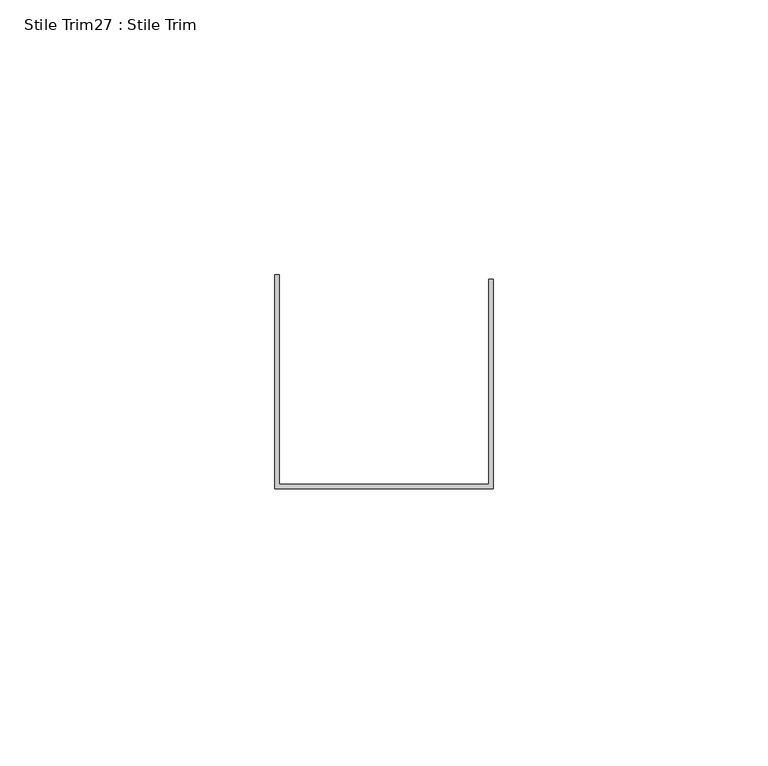
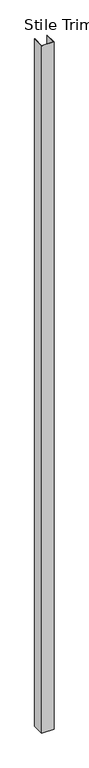
"""IFC4 building model written with IfcOpenShell, lengths in millimetres: proxy geometry, Stile Trim27 : Stile Trim."""

from ifc_helpers import new_model, si_unit, frame, origin, place, context, project, spatial, polyline, outline, extrude, source, transform, mapped, element, save


def stile_trim27_stile_trim_2fa88a95(model_context):
    return source(origin(), model_context, "Body", "SweptSolid", [
        extrude(outline(polyline([(587327.0060739, -535202.3537841), (587327.0060739, -535163.4663841), (587327.7934739, -535163.4663841), (587327.7934739, -535201.5663841), (587365.8934739, -535201.5663841), (587365.8934739, -535164.2537841), (587366.6808739, -535164.2537841), (587366.6808739, -535202.3537841), (587327.0060739, -535202.3537841)])), frame((0.0, 0.0, 50.8), z_axis=(0.0, 0.0, 1.0), x_axis=(1.0, 0.0, 0.0)), (0.0, 0.0, 1.0), 2350.3929688),
    ])


if __name__ == "__main__":
    model = new_model("IFC4")
    model_context = context("Model", 3, world=origin())
    ifc_project = project(units=[si_unit("LENGTHUNIT", "METRE", prefix="MILLI")], contexts=[model_context])
    site = spatial("IfcSite", under=ifc_project)
    building = spatial("IfcBuilding", under=site)
    placement = place(None, origin())
    stile_trim27_stile_trim_shape = stile_trim27_stile_trim_2fa88a95(model_context)
    element("IfcBuildingElementProxy", 1, Name="Stile Trim27 : Stile Trim", ObjectType="Stile Trim27 : Stile Trim", at=placement, inside=building, context=model_context, shape_type="MappedRepresentation", body=[
        mapped(stile_trim27_stile_trim_shape, transform((0.0, 0.0, 0.0), x_axis=(1.0, 0.0, 0.0), y_axis=(0.0, 1.0, 0.0), z_axis=(0.0, 0.0, 1.0))),
    ])
    save(model, "model.ifc")

# Revit data of these elements
# Element 1 (IfcBuildingElementProxy, "Stile Trim27 : Stile Trim")
#   Materials on its faces: "EDGE TRIM BY MTL PANEL MFR."
# Materials
#   "EDGE TRIM BY MTL PANEL MFR.": class "Generic", colour RGB 239 242 240, transparency 0, Cost = 0
